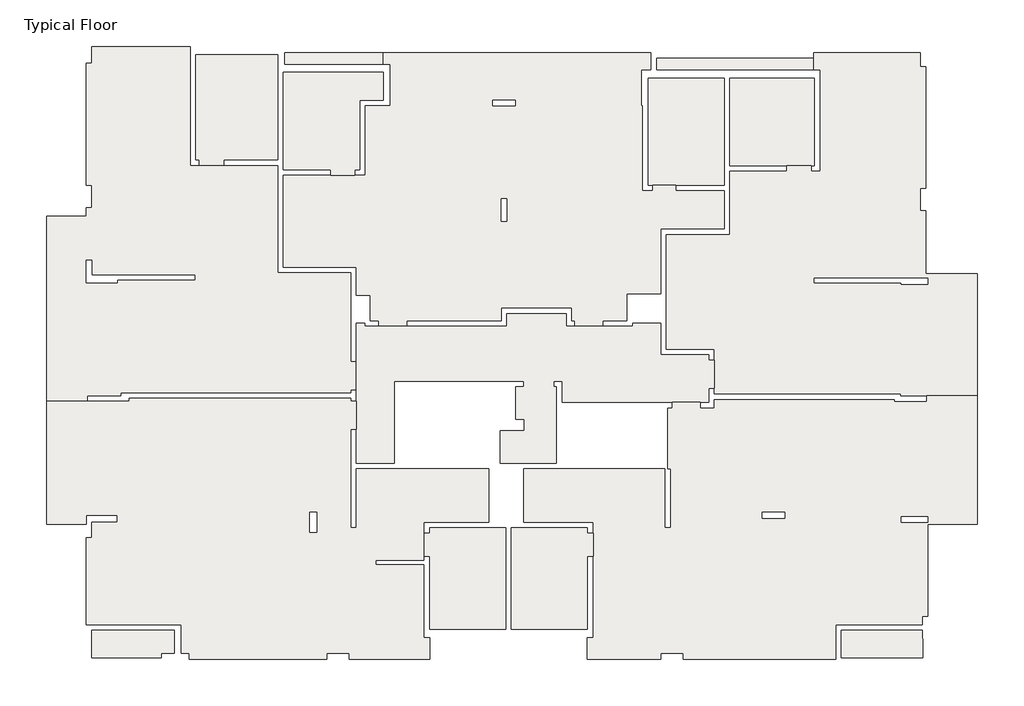
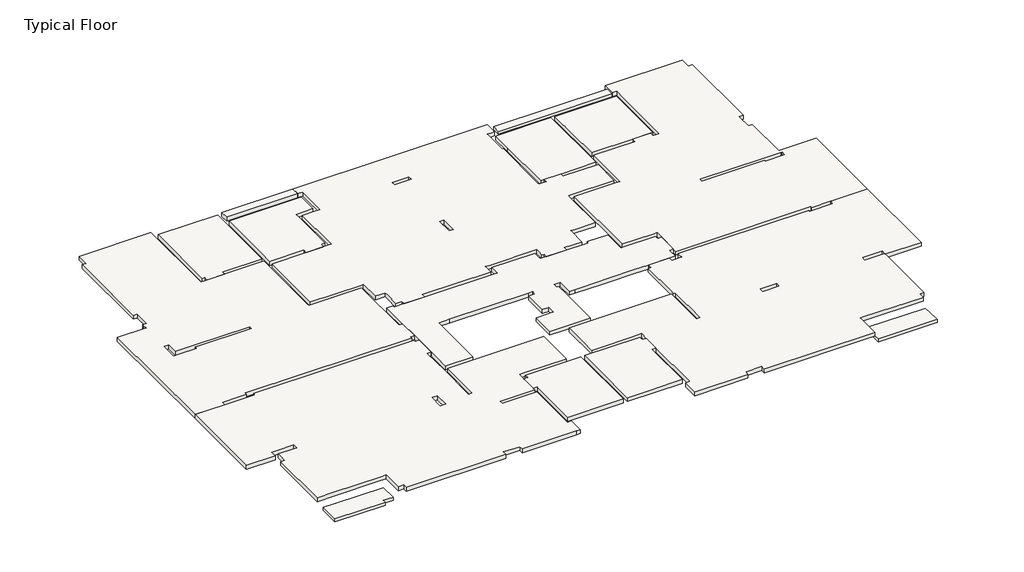
# One storey: 16 slabs.
"""IFC4 building model written with IfcOpenShell, lengths in millimetres."""

import ifcopenshell
import ifcopenshell.guid

model = None  # the IFC model being written
_history = None  # IfcOwnerHistory: only IFC2X3 demands one
_inside = {}  # id of a spatial element -> (the spatial element, [elements in it])
_under = {}  # id of a project, library or spatial element -> (it, [spatial elements below it])
_declared = {}  # id of a project -> (the project, [libraries it declares])
_typed = {}  # id of a type object -> (the type object, [elements of that type])
_made_of = {}  # id of a material, layer set ... -> (it, [elements and type objects made of it])


def new_model(schema):
    """Start an empty IFC model of exactly this schema.

    Asked for "IFC4X3", IfcOpenShell would pick the latest addendum, in which some entities
    have other attributes; the version numbers below select the first issue.
    IFC2X3 requires an IfcOwnerHistory on every rooted entity: one is made here for all.
    """
    global model, _history
    if schema == "IFC4X3":
        model = ifcopenshell.file(schema_version=(4, 3, 0, 0))
    else:
        model = ifcopenshell.file(schema=schema)
    _inside.clear()
    _under.clear()
    _declared.clear()
    _typed.clear()
    _made_of.clear()
    _history = None
    if model.schema == "IFC2X3":
        org = make("IfcOrganization", Name="unknown")
        user = make(
            "IfcPersonAndOrganization",
            ThePerson=make("IfcPerson", FamilyName="unknown"),
            TheOrganization=org,
        )
        app = make(
            "IfcApplication",
            ApplicationDeveloper=org,
            Version="unknown",
            ApplicationFullName="unknown",
            ApplicationIdentifier="unknown",
        )
        _history = make(
            "IfcOwnerHistory",
            OwningUser=user,
            OwningApplication=app,
            ChangeAction="ADDED",
            CreationDate=0,
        )
    return model


def make(cls, **values):
    """One entity of the class cls with the attributes given. An attribute that is None is left unset."""
    return model.create_entity(
        cls, **{name: value for name, value in values.items() if value is not None}
    )


def rooted(cls, **values):
    """An entity with a GlobalId (a new one), such as an element, a storey or a relation."""
    return make(cls, GlobalId=ifcopenshell.guid.new(), OwnerHistory=_history, **values)


def si_unit(unit_type, name, prefix=None):
    """IfcSIUnit, for example si_unit("LENGTHUNIT", "METRE", prefix="MILLI")."""
    return make("IfcSIUnit", UnitType=unit_type, Prefix=prefix, Name=name)


def assignment(units):
    """IfcUnitAssignment: the units of a project."""
    return None if units is None else make("IfcUnitAssignment", Units=units)


def point(xyz):
    """IfcCartesianPoint."""
    return None if xyz is None else make("IfcCartesianPoint", Coordinates=xyz)


def direction(xyz):
    """IfcDirection."""
    return None if xyz is None else make("IfcDirection", DirectionRatios=xyz)


def frame(location, z_axis=None, x_axis=None):
    """IfcAxis2Placement3D, a coordinate frame: its origin and axes. An axis left out is left unset."""
    return make(
        "IfcAxis2Placement3D",
        Location=point(location),
        Axis=direction(z_axis),
        RefDirection=direction(x_axis),
    )


def origin():
    """The frame at (0, 0, 0) with its axes left unset."""
    return frame((0.0, 0.0, 0.0))


def place(relative_to, where):
    """IfcLocalPlacement: puts the frame where relative to a parent placement (None: the world)."""
    return make(
        "IfcLocalPlacement", PlacementRelTo=relative_to, RelativePlacement=where
    )


def context(
    kind, dimensions, precision=None, world=None, true_north=None, identifier=None
):
    """IfcGeometricRepresentationContext, for example the 3D "Model" context."""
    return make(
        "IfcGeometricRepresentationContext",
        ContextIdentifier=identifier,
        ContextType=kind,
        CoordinateSpaceDimension=dimensions,
        Precision=precision,
        WorldCoordinateSystem=world,
        TrueNorth=true_north,
    )


def project(units=None, contexts=None):
    """IfcProject with its units and contexts."""
    return rooted(
        "IfcProject",
        Name="project",
        RepresentationContexts=contexts,
        UnitsInContext=assignment(units),
    )


def spatial(cls, under=None, at=None, **own):
    """A site, building, storey or space (cls), placed at a placement, below another one or the project."""
    s = rooted(cls, ObjectPlacement=at, **own)
    if under is not None:
        _under.setdefault(under.id(), (under, []))[1].append(s)
    return s


def polyline(points):
    """IfcPolyline through the points."""
    return make("IfcPolyline", Points=[point(p) for p in points])


def outline(outer, holes=None, kind="AREA"):
    """IfcArbitraryClosedProfileDef: a profile drawn as a closed curve; with holes, ...WithVoids."""
    if holes is None:
        return make("IfcArbitraryClosedProfileDef", ProfileType=kind, OuterCurve=outer)
    return make(
        "IfcArbitraryProfileDefWithVoids",
        ProfileType=kind,
        OuterCurve=outer,
        InnerCurves=holes,
    )


def extrude(swept, where, along, depth):
    """IfcExtrudedAreaSolid: the profile swept, set in the frame where, extruded along a direction by depth."""
    return make(
        "IfcExtrudedAreaSolid",
        SweptArea=swept,
        Position=where,
        ExtrudedDirection=direction(along),
        Depth=depth,
    )


def faces_of(points, faces, orient=None, outer=None):
    """IfcFace entities. A face is a list of loops; a loop is a list of indices into points, from 0.

    orient and outer hold one flag for each loop. By default every Orientation is true, the
    first loop of a face is its IfcFaceOuterBound and the others are IfcFaceBound.
    """
    made = []
    for i, loops in enumerate(faces):
        bounds = []
        for j, loop in enumerate(loops):
            is_outer = j == 0 if outer is None else outer[i][j]
            bounds.append(
                make(
                    "IfcFaceOuterBound" if is_outer else "IfcFaceBound",
                    Bound=make("IfcPolyLoop", Polygon=[points[k] for k in loop]),
                    Orientation=True if orient is None else orient[i][j],
                )
            )
        made.append(make("IfcFace", Bounds=bounds))
    return made


def faceted_brep(points, faces, orient=None, outer=None, voids=None):
    """IfcFacetedBrep: a solid bounded by flat faces; with voids (closed shells), ...WithVoids."""
    shared = [point(p) for p in points]
    hull = make("IfcClosedShell", CfsFaces=faces_of(shared, faces, orient, outer))
    if voids is None:
        return make("IfcFacetedBrep", Outer=hull)
    return make(
        "IfcFacetedBrepWithVoids",
        Outer=hull,
        Voids=[
            make(cls, CfsFaces=faces_of(shared, fs, o, b)) for cls, fs, o, b in voids
        ],
    )


def shape(context_of_items, identifier, shape_type, items):
    """IfcShapeRepresentation: the items that make up one representation, for example the "Body"."""
    return make(
        "IfcShapeRepresentation",
        ContextOfItems=context_of_items,
        RepresentationIdentifier=identifier,
        RepresentationType=shape_type,
        Items=items,
    )


def made_of(thing, what):
    """Note that an element or type object is made of a material, layer set ...; save() writes the relation."""
    if what is not None:
        _made_of.setdefault(what.id(), (what, []))[1].append(thing)
    return thing


def element(
    cls,
    number,
    at=None,
    inside=None,
    cuts=None,
    type_object=None,
    material=None,
    context=None,
    identifier="Body",
    shape_type=None,
    held_by="IfcProductDefinitionShape",
    body=None,
    shapes=None,
    **own,
):
    """One element of the class cls, such as IfcWall. Its Tag is "e" and its number.

    at: its placement. inside: the storey or other place that contains it. cuts: it is an
    opening in that element (IfcRelVoidsElement). A single representation is given by context,
    identifier, shape_type and body (its items); several are given by shapes. held_by: the class
    of the entity that holds the representations. save() writes the other relations.
    """
    e = rooted(cls, Tag="e%d" % number, ObjectPlacement=at, **own)
    if body is not None:
        shapes = [shape(context, identifier, shape_type, body)]
    if shapes is not None:
        e.Representation = make(held_by, Representations=shapes)
    if inside is not None:
        _inside.setdefault(inside.id(), (inside, []))[1].append(e)
    if cuts is not None:
        rooted(
            "IfcRelVoidsElement", RelatingBuildingElement=cuts, RelatedOpeningElement=e
        )
    if type_object is not None:
        _typed.setdefault(type_object.id(), (type_object, []))[1].append(e)
    return made_of(e, material)


def aggregate(whole, parts):
    """IfcRelAggregates: a whole, such as a stair, and the parts it consists of."""
    return rooted("IfcRelAggregates", RelatingObject=whole, RelatedObjects=parts)


def save(model, path):
    """Write the relations noted so far, then the file.

    IfcRelAggregates (storeys below a building ...), IfcRelContainedInSpatialStructure (elements
    in a storey), IfcRelDefinesByType, IfcRelAssociatesMaterial and IfcRelDeclares: one each for
    every whole, place, type object, material and project.
    """
    for whole, parts in _under.values():
        aggregate(whole, parts)
    for where, things in _inside.values():
        rooted(
            "IfcRelContainedInSpatialStructure",
            RelatedElements=things,
            RelatingStructure=where,
        )
    for kind, things in _typed.values():
        rooted("IfcRelDefinesByType", RelatedObjects=things, RelatingType=kind)
    for what, things in _made_of.values():
        rooted("IfcRelAssociatesMaterial", RelatedObjects=things, RelatingMaterial=what)
    for by, libraries in _declared.values():
        rooted("IfcRelDeclares", RelatingContext=by, RelatedDefinitions=libraries)
    model.write(path)


model = new_model("IFC4")

# Units and contexts
model_context = context("Model", 3, world=origin())
ifc_project = project(units=[si_unit("LENGTHUNIT", "METRE", prefix="MILLI")], contexts=[model_context])

# Site, building, storey
site = spatial("IfcSite", under=ifc_project)
building = spatial("IfcBuilding", under=site)
storey = spatial("IfcBuildingStorey", under=building, Name="Typical Floor", Elevation=3270.0)

# Slabs
placement = place(None, origin())
element("IfcSlab", 1, ObjectType="15", at=placement, inside=storey, context=model_context, shape_type="Brep", body=[
    faceted_brep([(-21571.9643546, 17066.3078446, 2670.0), (-24032.496199, 17066.3078446, 2670.0), (-24034.296226, 17066.3078446, 2670.0), (-24034.296226, 18036.7796078, 2670.0), (-23432.496199, 18036.7796078, 2670.0), (-23432.496199, 18038.5478478, 2670.0), (-21102.3452666, 18038.5478478, 2670.0), (-21102.3452666, 17215.5200253, 2670.0), (-21571.9643546, 17215.5200253, 2670.0), (-24034.296226, 17066.3078446, 2820.0), (-24032.496199, 17066.3078446, 2820.0), (-21571.9643546, 17066.3078446, 2820.0), (-21571.9643546, 17215.5200253, 2820.0), (-21102.3452666, 17215.5200253, 2820.0), (-21102.3452666, 18036.7796078, 2820.0), (-21102.3452666, 18038.5478478, 2820.0), (-23432.496199, 18038.5478478, 2820.0), (-23432.496199, 18036.7796078, 2820.0), (-24032.496199, 18036.7796078, 2820.0), (-24034.296226, 18036.7796078, 2820.0)], [[[0, 1, 2, 3, 4, 5, 6, 7, 8]], [[9, 10, 11, 12, 13, 14, 15, 16, 17, 18, 19]], [[11, 0, 8, 12]], [[2, 1, 0, 11, 10, 9]], [[2, 9, 19, 3]], [[15, 6, 5, 16]], [[7, 6, 15, 14, 13]], [[12, 8, 7, 13]], [[4, 17, 16, 5]], [[17, 4, 3, 19, 18]]]),
])
element("IfcSlab", 2, ObjectType="15", at=placement, inside=storey, context=model_context, shape_type="Brep", body=[
    faceted_brep([(5430.732608, 17066.3078446, 2670.0), (5420.732608, 17066.3078446, 2670.0), (2546.318889, 17066.3078446, 2670.0), (2541.318889, 17066.3078446, 2670.0), (2541.318889, 17435.7075634, 2670.0), (2546.318889, 17435.7075634, 2670.0), (2546.318889, 18040.7075634, 2670.0), (5420.732608, 18040.7075634, 2670.0), (5420.732608, 17735.2006534, 2670.0), (5430.732608, 17735.2006534, 2670.0), (2541.318889, 17066.3078446, 2820.0), (2546.318889, 17066.3078446, 2820.0), (5420.732608, 17066.3078446, 2820.0), (5430.732608, 17066.3078446, 2820.0), (5430.732608, 17735.2006534, 2820.0), (5420.732608, 17735.2006534, 2820.0), (5420.732608, 18035.7075634, 2820.0), (5420.732608, 18040.7075634, 2820.0), (2546.318889, 18040.7075634, 2820.0), (2546.318889, 18035.7075634, 2820.0), (2546.318889, 17435.7075634, 2820.0), (2541.318889, 17435.7075634, 2820.0)], [[[0, 1, 2, 3, 4, 5, 6, 7, 8, 9]], [[10, 11, 12, 13, 14, 15, 16, 17, 18, 19, 20, 21]], [[3, 2, 1, 0, 13, 12, 11, 10]], [[3, 10, 21, 4]], [[6, 18, 17, 7]], [[13, 0, 9, 14]], [[5, 20, 19, 18, 6]], [[20, 5, 4, 21]], [[8, 15, 14, 9]], [[15, 8, 7, 17, 16]]]),
])
element("IfcSlab", 3, ObjectType="15", at=placement, inside=storey, context=model_context, shape_type="SweptSolid", body=[
    extrude(outline(polyline([(1566.3525769, 38314.4998391), (1566.3525769, 37914.469069), (-4002.3443382, 37914.469069), (-4002.3443382, 38314.4998391), (1566.3525769, 38314.4998391)])), frame((0.0, 0.0, 3070.0), z_axis=(0.0, 0.0, 1.0), x_axis=(1.0, 0.0, 0.0)), (0.0, 0.0, 1.0), 150.0),
])
element("IfcSlab", 4, ObjectType="20", at=placement, inside=storey, context=model_context, shape_type="Brep", body=[
    faceted_brep([(1597.1133398, 37614.469069, 3070.0), (1597.1133398, 34516.3054573, 3070.0), (1475.3435315, 34516.3054573, 3070.0), (620.1311917, 34516.3054573, 3070.0), (-1403.2009922, 34516.3054573, 3070.0), (-1403.2009922, 37614.469069, 3070.0), (1597.1133398, 37614.469069, 3270.0), (-1403.2009922, 37614.469069, 3270.0), (-1403.2009922, 34516.3054573, 3270.0), (620.1311917, 34516.3054573, 3270.0), (1475.3435315, 34516.3054573, 3270.0), (1597.1133398, 34516.3054573, 3270.0)], [[[0, 1, 2, 3, 4, 5]], [[6, 7, 8, 9, 10, 11]], [[1, 0, 6, 11]], [[4, 3, 2, 1, 11, 10, 9, 8]], [[5, 4, 8, 7]], [[0, 5, 7, 6]]]),
])
element("IfcSlab", 5, ObjectType="20", at=placement, inside=storey, context=model_context, shape_type="Brep", body=[
    faceted_brep([(-1603.2009922, 37614.469069, 3070.0), (-1603.2009922, 33815.7403229, 3070.0), (-3320.8331575, 33815.7403229, 3070.0), (-4138.8749491, 33815.7403229, 3070.0), (-4301.8715139, 33815.7403229, 3070.0), (-4301.8715139, 36636.0817113, 3070.0), (-4302.6593333, 36636.0817113, 3070.0), (-4302.6593333, 37614.469069, 3070.0), (-1603.2009922, 33815.7403229, 3270.0), (-1603.2009922, 37614.469069, 3270.0), (-4302.6593333, 37614.469069, 3270.0), (-4302.6593333, 36636.0817113, 3270.0), (-4301.8715139, 36636.0817113, 3270.0), (-4301.8715139, 33815.7403229, 3270.0), (-4138.8749491, 33815.7403229, 3270.0), (-3320.8331575, 33815.7403229, 3270.0)], [[[0, 1, 2, 3, 4, 5, 6, 7]], [[8, 9, 10, 11, 12, 13, 14, 15]], [[1, 0, 9, 8]], [[1, 8, 15, 14, 13, 4, 3, 2]], [[10, 7, 6, 11]], [[0, 7, 10, 9]], [[12, 5, 4, 13]], [[5, 12, 11, 6]]]),
])
element("IfcSlab", 6, ObjectType="20", at=placement, inside=storey, context=model_context, shape_type="Brep", body=[
    faceted_brep([(1566.3525769, 37914.469069, 3070.0), (1566.3525769, 38314.4998391, 3070.0), (1566.3525769, 38515.575292, 3070.0), (5346.4978686, 38515.575292, 3070.0), (5346.4978686, 38016.0787934, 3070.0), (5546.4978686, 38016.0787934, 3070.0), (5546.4978686, 33715.2026429, 3070.0), (5346.4978686, 33715.2026429, 3070.0), (5346.4978686, 32915.2026429, 3070.0), (5546.4978686, 32915.2026429, 3070.0), (5546.4978686, 30686.4079799, 3070.0), (5547.5722379, 30686.4079799, 3070.0), (7376.2745907, 30686.4079799, 3070.0), (7376.2745907, 26346.3859634, 3070.0), (5607.1364173, 26346.3859634, 3070.0), (5577.2268706, 26346.3859634, 3070.0), (4656.569824, 26346.3859634, 3070.0), (4656.569824, 26415.1864621, 3070.0), (-1953.6864162, 26415.1864621, 3070.0), (-1953.6864162, 26616.2585064, 3070.0), (-1953.6864162, 27615.2787722, 3070.0), (-1953.6864162, 28004.6755732, 3070.0), (-2153.6864162, 28004.6755732, 3070.0), (-3652.0941989, 28004.6755732, 3070.0), (-3652.0941989, 32066.405062, 3070.0), (-1603.2009922, 32066.405062, 3070.0), (-1403.2009922, 32066.405062, 3070.0), (-1403.2009922, 34316.3054573, 3070.0), (620.1311917, 34316.3054573, 3070.0), (620.1311917, 34516.3054573, 3070.0), (1475.3435315, 34516.3054573, 3070.0), (1475.3435315, 34316.3054573, 3070.0), (1797.1133398, 34316.3054573, 3070.0), (1797.1133398, 34516.3054573, 3070.0), (1797.1133398, 37614.469069, 3070.0), (1797.1133398, 37914.469069, 3070.0), (1598.0523567, 30514.7063432, 3070.0), (1598.0523567, 30364.7063432, 3070.0), (4667.1364173, 30364.7063432, 3070.0), (4667.1364173, 30314.7063432, 3070.0), (5607.1364173, 30314.7063432, 3070.0), (5607.1364173, 30514.7063432, 3070.0), (5546.4978686, 30514.7063432, 3070.0), (4667.1364173, 30514.7063432, 3070.0), (1566.3525769, 38515.575292, 3270.0), (1566.3525769, 37914.469069, 3270.0), (1797.1133398, 37914.469069, 3270.0), (1797.1133398, 37614.469069, 3270.0), (1797.1133398, 34516.3054573, 3270.0), (1797.1133398, 34316.3054573, 3270.0), (1475.3435315, 34316.3054573, 3270.0), (1475.3435315, 34516.3054573, 3270.0), (620.1311917, 34516.3054573, 3270.0), (620.1311917, 34316.3054573, 3270.0), (-1403.2009922, 34316.3054573, 3270.0), (-1403.2009922, 32066.405062, 3270.0), (-1603.2009922, 32066.405062, 3270.0), (-3652.0941989, 32066.405062, 3270.0), (-3652.0941989, 28004.6755732, 3270.0), (-2153.6864162, 28004.6755732, 3270.0), (-1953.6864162, 28004.6755732, 3270.0), (-1953.6864162, 27615.2787722, 3270.0), (-1953.6864162, 26616.2585064, 3270.0), (-1953.6864162, 26415.1864621, 3270.0), (4656.569824, 26415.1864621, 3270.0), (4656.569824, 26346.3859634, 3270.0), (5577.2268706, 26346.3859634, 3270.0), (5607.1364173, 26346.3859634, 3270.0), (7376.2745907, 26346.3859634, 3270.0), (7376.2745907, 30686.4079799, 3270.0), (5546.4978686, 30686.4079799, 3270.0), (5546.4978686, 32915.2026429, 3270.0), (5346.4978686, 32915.2026429, 3270.0), (5346.4978686, 33715.2026429, 3270.0), (5546.4978686, 33715.2026429, 3270.0), (5546.4978686, 38016.0787934, 3270.0), (5346.4978686, 38016.0787934, 3270.0), (5346.4978686, 38515.575292, 3270.0), (1598.0523567, 30364.7063432, 3270.0), (1598.0523567, 30514.7063432, 3270.0), (4667.1364173, 30514.7063432, 3270.0), (5546.4978686, 30514.7063432, 3270.0), (5607.1364173, 30514.7063432, 3270.0), (5607.1364173, 30314.7063432, 3270.0), (4667.1364173, 30314.7063432, 3270.0), (4667.1364173, 30364.7063432, 3270.0), (1566.3525769, 37914.469069, 3220.0)], [[[0, 1, 2, 3, 4, 5, 6, 7, 8, 9, 10, 11, 12, 13, 14, 15, 16, 17, 18, 19, 20, 21, 22, 23, 24, 25, 26, 27, 28, 29, 30, 31, 32, 33, 34, 35], [36, 37, 38, 39, 40, 41, 42, 43]], [[44, 45, 46, 47, 48, 49, 50, 51, 52, 53, 54, 55, 56, 57, 58, 59, 60, 61, 62, 63, 64, 65, 66, 67, 68, 69, 70, 71, 72, 73, 74, 75, 76, 77], [78, 79, 80, 81, 82, 83, 84, 85]], [[2, 1, 0, 86, 45, 44]], [[3, 2, 44, 77]], [[4, 3, 77, 76]], [[5, 4, 76, 75]], [[6, 5, 75, 74]], [[7, 6, 74, 73]], [[8, 7, 73, 72]], [[9, 8, 72, 71]], [[10, 9, 71, 70]], [[79, 36, 43, 42, 81, 80]], [[37, 36, 79, 78]], [[38, 37, 78, 85]], [[39, 38, 85, 84]], [[40, 39, 84, 83]], [[16, 15, 14, 67, 66, 65]], [[17, 16, 65, 64]], [[18, 17, 64, 63]], [[19, 18, 63, 62]], [[20, 19, 62, 61]], [[21, 20, 61, 60]], [[21, 60, 59, 58, 23, 22]], [[24, 23, 58, 57]], [[24, 57, 56, 55, 26, 25]], [[27, 26, 55, 54]], [[28, 27, 54, 53]], [[29, 28, 53, 52]], [[30, 29, 52, 51]], [[31, 30, 51, 50]], [[32, 31, 50, 49]], [[32, 49, 48, 47, 46, 35, 34, 33]], [[0, 35, 46, 45, 86]], [[12, 11, 10, 70, 69]], [[13, 12, 69, 68]], [[14, 13, 68, 67]], [[41, 40, 83, 82]], [[42, 41, 82, 81]]]),
])
element("IfcSlab", 7, ObjectType="20", at=placement, inside=storey, context=model_context, shape_type="Brep", body=[
    faceted_brep([(-1953.6864162, 27615.2787722, 3070.0), (-1953.6864162, 26616.2585064, 3070.0), (-2153.6864162, 26616.2585064, 3070.0), (-2153.6864162, 26116.7313306, 3070.0), (-2453.0431631, 26116.7313306, 3070.0), (-3452.0634289, 26116.7313306, 3070.0), (-4152.6285632, 26116.7313306, 3070.0), (-5452.2172791, 26116.7313306, 3070.0), (-5750.6383247, 26116.7313306, 3070.0), (-7052.3403593, 26116.7313306, 3070.0), (-7352.8747236, 26116.7313306, 3070.0), (-7352.8747236, 26666.0050514, 3070.0), (-7352.8747236, 26866.0050514, 3070.0), (-7653.4431737, 26866.0050514, 3070.0), (-7653.4431737, 26666.0050514, 3070.0), (-7552.8747236, 26666.0050514, 3070.0), (-7552.8747236, 26116.7313306, 3070.0), (-7552.8747236, 25916.7313306, 3070.0), (-7552.8747236, 23965.2552968, 3070.0), (-9538.2512588, 23965.2552968, 3070.0), (-9538.2512588, 25114.9330071, 3070.0), (-8698.2512588, 25114.9330071, 3070.0), (-8698.2512588, 25514.9330071, 3070.0), (-9003.2512588, 25514.9330071, 3070.0), (-9003.2512588, 26664.9330071, 3070.0), (-8703.2512588, 26664.9330071, 3070.0), (-8703.2512588, 26864.9330071, 3070.0), (-8902.548455, 26864.9330071, 3070.0), (-12762.548455, 26864.9330071, 3070.0), (-13303.2512588, 26864.9330071, 3070.0), (-13303.2512588, 26664.9330071, 3070.0), (-13302.548455, 26664.9330071, 3070.0), (-13302.548455, 23965.2552968, 3070.0), (-14651.8837159, 23965.2552968, 3070.0), (-14651.8837159, 25164.3063326, 3070.0), (-14652.9249902, 25164.3063326, 3070.0), (-14652.9249902, 26165.4399171, 3070.0), (-14652.9249902, 26561.209964, 3070.0), (-14652.9249902, 27566.6042716, 3070.0), (-14652.9249902, 28915.3710824, 3070.0), (-14353.3978144, 28915.3710824, 3070.0), (-14353.3978144, 28815.3710824, 3070.0), (-13852.8634501, 28815.3710824, 3070.0), (-12851.7298656, 28815.3710824, 3070.0), (-9317.0680709, 28815.3710824, 3070.0), (-9317.0680709, 29015.3710824, 3070.0), (-9317.0680709, 29265.1483974, 3070.0), (-7203.6658586, 29265.1483974, 3070.0), (-7203.6658586, 29015.3710824, 3070.0), (-7203.6658586, 28815.3710824, 3070.0), (-6902.0561342, 28815.3710824, 3070.0), (-5903.0358684, 28815.3710824, 3070.0), (-4853.2277833, 28815.3710824, 3070.0), (-4853.2277833, 28914.6755732, 3070.0), (-3852.0941989, 28914.6755732, 3070.0), (-3852.0941989, 27804.6755732, 3070.0), (-3652.0941989, 27804.6755732, 3070.0), (-2153.6864162, 27804.6755732, 3070.0), (-2153.6864162, 27615.2787722, 3070.0), (-1953.6864162, 26616.2585064, 3270.0), (-1953.6864162, 27615.2787722, 3270.0), (-2153.6864162, 27615.2787722, 3270.0), (-2153.6864162, 27804.6755732, 3270.0), (-3652.0941989, 27804.6755732, 3270.0), (-3852.0941989, 27804.6755732, 3270.0), (-3852.0941989, 28914.6755732, 3270.0), (-4853.2277833, 28914.6755732, 3270.0), (-4853.2277833, 28815.3710824, 3270.0), (-5903.0358684, 28815.3710824, 3270.0), (-6902.0561342, 28815.3710824, 3270.0), (-7203.6658586, 28815.3710824, 3270.0), (-7203.6658586, 29015.3710824, 3270.0), (-7203.6658586, 29265.1483974, 3270.0), (-9317.0680709, 29265.1483974, 3270.0), (-9317.0680709, 29015.3710824, 3270.0), (-9317.0680709, 28815.3710824, 3270.0), (-12851.7298656, 28815.3710824, 3270.0), (-13852.8634501, 28815.3710824, 3270.0), (-14353.3978144, 28815.3710824, 3270.0), (-14353.3978144, 28915.3710824, 3270.0), (-14652.9249902, 28915.3710824, 3270.0), (-14652.9249902, 27566.6042716, 3270.0), (-14652.9249902, 26561.209964, 3270.0), (-14652.9249902, 26165.4399171, 3270.0), (-14652.9249902, 25164.3063326, 3270.0), (-14651.8837159, 25164.3063326, 3270.0), (-14651.8837159, 23965.2552968, 3270.0), (-13302.548455, 23965.2552968, 3270.0), (-13302.548455, 26664.9330071, 3270.0), (-13303.2512588, 26664.9330071, 3270.0), (-13303.2512588, 26864.9330071, 3270.0), (-12762.548455, 26864.9330071, 3270.0), (-8902.548455, 26864.9330071, 3270.0), (-8703.2512588, 26864.9330071, 3270.0), (-8703.2512588, 26664.9330071, 3270.0), (-9003.2512588, 26664.9330071, 3270.0), (-9003.2512588, 25514.9330071, 3270.0), (-8698.2512588, 25514.9330071, 3270.0), (-8698.2512588, 25114.9330071, 3270.0), (-9538.2512588, 25114.9330071, 3270.0), (-9538.2512588, 23965.2552968, 3270.0), (-7552.8747236, 23965.2552968, 3270.0), (-7552.8747236, 25916.7313306, 3270.0), (-7552.8747236, 26116.7313306, 3270.0), (-7552.8747236, 26666.0050514, 3270.0), (-7653.4431737, 26666.0050514, 3270.0), (-7653.4431737, 26866.0050514, 3270.0), (-7352.8747236, 26866.0050514, 3270.0), (-7352.8747236, 26666.0050514, 3270.0), (-7352.8747236, 26116.7313306, 3270.0), (-7052.3403593, 26116.7313306, 3270.0), (-5750.6383247, 26116.7313306, 3270.0), (-5452.2172791, 26116.7313306, 3270.0), (-4152.6285632, 26116.7313306, 3270.0), (-3452.0634289, 26116.7313306, 3270.0), (-2453.0431631, 26116.7313306, 3270.0), (-2153.6864162, 26116.7313306, 3270.0), (-2153.6864162, 26616.2585064, 3270.0)], [[[0, 1, 2, 3, 4, 5, 6, 7, 8, 9, 10, 11, 12, 13, 14, 15, 16, 17, 18, 19, 20, 21, 22, 23, 24, 25, 26, 27, 28, 29, 30, 31, 32, 33, 34, 35, 36, 37, 38, 39, 40, 41, 42, 43, 44, 45, 46, 47, 48, 49, 50, 51, 52, 53, 54, 55, 56, 57, 58]], [[59, 60, 61, 62, 63, 64, 65, 66, 67, 68, 69, 70, 71, 72, 73, 74, 75, 76, 77, 78, 79, 80, 81, 82, 83, 84, 85, 86, 87, 88, 89, 90, 91, 92, 93, 94, 95, 96, 97, 98, 99, 100, 101, 102, 103, 104, 105, 106, 107, 108, 109, 110, 111, 112, 113, 114, 115, 116, 117]], [[1, 0, 60, 59]], [[2, 1, 59, 117]], [[3, 2, 117, 116]], [[3, 116, 115, 114, 5, 4]], [[5, 114, 113, 112, 111, 110, 9, 8, 7, 6]], [[10, 9, 110, 109]], [[10, 109, 108, 107, 12, 11]], [[13, 12, 107, 106]], [[14, 13, 106, 105]], [[15, 14, 105, 104]], [[15, 104, 103, 102, 101, 18, 17, 16]], [[19, 18, 101, 100]], [[20, 19, 100, 99]], [[21, 20, 99, 98]], [[22, 21, 98, 97]], [[23, 22, 97, 96]], [[24, 23, 96, 95]], [[25, 24, 95, 94]], [[26, 25, 94, 93]], [[27, 26, 93, 92]], [[28, 27, 92, 91]], [[28, 91, 90, 29]], [[87, 32, 31, 88]], [[33, 32, 87, 86]], [[34, 33, 86, 85]], [[35, 34, 85, 84]], [[36, 35, 84, 83]], [[37, 36, 83, 82]], [[38, 37, 82, 81]], [[39, 38, 81, 80]], [[40, 39, 80, 79]], [[41, 40, 79, 78]], [[42, 41, 78, 77]], [[43, 42, 77, 76]], [[44, 43, 76, 75]], [[44, 75, 74, 73, 46, 45]], [[47, 46, 73, 72]], [[47, 72, 71, 70, 49, 48]], [[50, 49, 70, 69]], [[51, 50, 69, 68]], [[52, 51, 68, 67]], [[53, 52, 67, 66]], [[54, 53, 66, 65]], [[55, 54, 65, 64]], [[55, 64, 63, 62, 57, 56]], [[58, 57, 62, 61]], [[0, 58, 61, 60]], [[30, 89, 88, 31]], [[29, 90, 89, 30]]]),
])
element("IfcSlab", 8, ObjectType="20", at=placement, inside=storey, context=model_context, shape_type="Brep", body=[
    faceted_brep([(-13700.7193614, 37815.0067491, 3070.0), (-13700.7193614, 36836.0817113, 3070.0), (-14532.2613121, 36836.0817113, 3070.0), (-14532.2613121, 36636.0817113, 3070.0), (-14532.2613121, 34366.055318, 3070.0), (-14705.8261281, 34366.055318, 3070.0), (-14705.8261281, 34166.055318, 3070.0), (-15560.9362106, 34166.055318, 3070.0), (-15560.9362106, 34366.055318, 3070.0), (-17231.9731082, 34366.055318, 3070.0), (-17231.9731082, 37815.0067491, 3070.0), (-13700.7193614, 36836.0817113, 3270.0), (-13700.7193614, 37815.0067491, 3270.0), (-17231.9731082, 37815.0067491, 3270.0), (-17231.9731082, 34366.055318, 3270.0), (-15560.9362106, 34366.055318, 3270.0), (-15560.9362106, 34166.055318, 3270.0), (-14705.8261281, 34166.055318, 3270.0), (-14705.8261281, 34366.055318, 3270.0), (-14532.2613121, 34366.055318, 3270.0), (-14532.2613121, 36636.0817113, 3270.0), (-14532.2613121, 36836.0817113, 3270.0)], [[[0, 1, 2, 3, 4, 5, 6, 7, 8, 9, 10]], [[11, 12, 13, 14, 15, 16, 17, 18, 19, 20, 21]], [[1, 0, 12, 11]], [[2, 1, 11, 21]], [[2, 21, 20, 19, 4, 3]], [[5, 4, 19, 18]], [[6, 5, 18, 17]], [[7, 6, 17, 16]], [[8, 7, 16, 15]], [[9, 8, 15, 14]], [[10, 9, 14, 13]], [[0, 10, 13, 12]]]),
])
element("IfcSlab", 9, ObjectType="20", at=placement, inside=storey, context=model_context, shape_type="Brep", body=[
    faceted_brep([(-13700.7193614, 38514.5374263, 3070.0), (-4202.3443382, 38514.5374263, 3070.0), (-4202.3443382, 37914.469069, 3070.0), (-4302.6593333, 37914.469069, 3070.0), (-4552.6593333, 37914.469069, 3070.0), (-4552.6593333, 36636.0817113, 3070.0), (-4501.8715139, 36636.0817113, 3070.0), (-4501.8715139, 33815.7403229, 3070.0), (-4501.8715139, 33615.7403229, 3070.0), (-4138.8749491, 33615.7403229, 3070.0), (-4138.8749491, 33815.7403229, 3070.0), (-3320.8331575, 33815.7403229, 3070.0), (-3320.8331575, 33615.7403229, 3070.0), (-1603.2009922, 33615.7403229, 3070.0), (-1603.2009922, 32266.405062, 3070.0), (-3852.0941989, 32266.405062, 3070.0), (-3852.0941989, 32066.405062, 3070.0), (-3852.0941989, 29964.6755732, 3070.0), (-4853.2277833, 29964.6755732, 3070.0), (-5053.2277833, 29964.6755732, 3070.0), (-5053.2277833, 29015.3710824, 3070.0), (-5903.0358684, 29015.3710824, 3070.0), (-5903.0358684, 28815.3710824, 3070.0), (-6902.0561342, 28815.3710824, 3070.0), (-6902.0561342, 29015.3710824, 3070.0), (-7003.6658586, 29015.3710824, 3070.0), (-7003.6658586, 29265.1483974, 3070.0), (-7003.6658586, 29465.1483974, 3070.0), (-9317.0680709, 29465.1483974, 3070.0), (-9517.0680709, 29465.1483974, 3070.0), (-9517.0680709, 29015.3710824, 3070.0), (-12851.7298656, 29015.3710824, 3070.0), (-12851.7298656, 28815.3710824, 3070.0), (-13852.8634501, 28815.3710824, 3070.0), (-13852.8634501, 29015.3710824, 3070.0), (-14153.3978144, 29015.3710824, 3070.0), (-14153.3978144, 29714.8949424, 3070.0), (-14153.3978144, 29914.8949424, 3070.0), (-14652.9249902, 29914.8949424, 3070.0), (-14652.9249902, 30914.9872525, 3070.0), (-14852.9249902, 30914.9872525, 3070.0), (-17231.9731082, 30914.9872525, 3070.0), (-17231.9731082, 34166.055318, 3070.0), (-15560.9362106, 34166.055318, 3070.0), (-14705.8261281, 34166.055318, 3070.0), (-14332.2613121, 34166.055318, 3070.0), (-14332.2613121, 34366.055318, 3070.0), (-14332.2613121, 36636.0817113, 3070.0), (-13700.7193614, 36636.0817113, 3070.0), (-13450.7193614, 36636.0817113, 3070.0), (-13450.7193614, 37815.0067491, 3070.0), (-13450.7193614, 38115.0067491, 3070.0), (-13700.7193614, 38115.0067491, 3070.0), (-9008.1078863, 36835.040437, 3070.0), (-9808.1078863, 36835.040437, 3070.0), (-9808.1078863, 36635.040437, 3070.0), (-9008.1078863, 36635.040437, 3070.0), (-9307.5394362, 33336.3391452, 3070.0), (-9507.5394362, 33336.3391452, 3070.0), (-9507.5394362, 32536.3391452, 3070.0), (-9307.5394362, 32536.3391452, 3070.0), (-4202.3443382, 38514.5374263, 3270.0), (-13700.7193614, 38514.5374263, 3270.0), (-13700.7193614, 38115.0067491, 3270.0), (-13450.7193614, 38115.0067491, 3270.0), (-13450.7193614, 37815.0067491, 3270.0), (-13450.7193614, 36636.0817113, 3270.0), (-13700.7193614, 36636.0817113, 3270.0), (-14332.2613121, 36636.0817113, 3270.0), (-14332.2613121, 34366.055318, 3270.0), (-14332.2613121, 34166.055318, 3270.0), (-14705.8261281, 34166.055318, 3270.0), (-15560.9362106, 34166.055318, 3270.0), (-17231.9731082, 34166.055318, 3270.0), (-17231.9731082, 30914.9872525, 3270.0), (-14852.9249902, 30914.9872525, 3270.0), (-14652.9249902, 30914.9872525, 3270.0), (-14652.9249902, 29914.8949424, 3270.0), (-14153.3978144, 29914.8949424, 3270.0), (-14153.3978144, 29714.8949424, 3270.0), (-14153.3978144, 29015.3710824, 3270.0), (-13852.8634501, 29015.3710824, 3270.0), (-13852.8634501, 28815.3710824, 3270.0), (-12851.7298656, 28815.3710824, 3270.0), (-12851.7298656, 29015.3710824, 3270.0), (-9517.0680709, 29015.3710824, 3270.0), (-9517.0680709, 29465.1483974, 3270.0), (-9317.0680709, 29465.1483974, 3270.0), (-7003.6658586, 29465.1483974, 3270.0), (-7003.6658586, 29265.1483974, 3270.0), (-7003.6658586, 29015.3710824, 3270.0), (-6902.0561342, 29015.3710824, 3270.0), (-6902.0561342, 28815.3710824, 3270.0), (-5903.0358684, 28815.3710824, 3270.0), (-5903.0358684, 29015.3710824, 3270.0), (-5053.2277833, 29015.3710824, 3270.0), (-5053.2277833, 29964.6755732, 3270.0), (-4853.2277833, 29964.6755732, 3270.0), (-3852.0941989, 29964.6755732, 3270.0), (-3852.0941989, 32066.405062, 3270.0), (-3852.0941989, 32266.405062, 3270.0), (-1603.2009922, 32266.405062, 3270.0), (-1603.2009922, 33615.7403229, 3270.0), (-3320.8331575, 33615.7403229, 3270.0), (-3320.8331575, 33815.7403229, 3270.0), (-4138.8749491, 33815.7403229, 3270.0), (-4138.8749491, 33615.7403229, 3270.0), (-4501.8715139, 33615.7403229, 3270.0), (-4501.8715139, 33815.7403229, 3270.0), (-4501.8715139, 36636.0817113, 3270.0), (-4552.6593333, 36636.0817113, 3270.0), (-4552.6593333, 37914.469069, 3270.0), (-4302.6593333, 37914.469069, 3270.0), (-4202.3443382, 37914.469069, 3270.0), (-9808.1078863, 36835.040437, 3270.0), (-9008.1078863, 36835.040437, 3270.0), (-9008.1078863, 36635.040437, 3270.0), (-9808.1078863, 36635.040437, 3270.0), (-9507.5394362, 33336.3391452, 3270.0), (-9307.5394362, 33336.3391452, 3270.0), (-9307.5394362, 32536.3391452, 3270.0), (-9507.5394362, 32536.3391452, 3270.0)], [[[0, 1, 2, 3, 4, 5, 6, 7, 8, 9, 10, 11, 12, 13, 14, 15, 16, 17, 18, 19, 20, 21, 22, 23, 24, 25, 26, 27, 28, 29, 30, 31, 32, 33, 34, 35, 36, 37, 38, 39, 40, 41, 42, 43, 44, 45, 46, 47, 48, 49, 50, 51, 52], [53, 54, 55, 56], [57, 58, 59, 60]], [[61, 62, 63, 64, 65, 66, 67, 68, 69, 70, 71, 72, 73, 74, 75, 76, 77, 78, 79, 80, 81, 82, 83, 84, 85, 86, 87, 88, 89, 90, 91, 92, 93, 94, 95, 96, 97, 98, 99, 100, 101, 102, 103, 104, 105, 106, 107, 108, 109, 110, 111, 112, 113], [114, 115, 116, 117], [118, 119, 120, 121]], [[1, 0, 62, 61]], [[2, 1, 61, 113]], [[2, 113, 112, 111, 4, 3]], [[5, 4, 111, 110]], [[6, 5, 110, 109]], [[6, 109, 108, 107, 8, 7]], [[9, 8, 107, 106]], [[10, 9, 106, 105]], [[11, 10, 105, 104]], [[12, 11, 104, 103]], [[13, 12, 103, 102]], [[14, 13, 102, 101]], [[15, 14, 101, 100]], [[15, 100, 99, 98, 17, 16]], [[17, 98, 97, 96, 19, 18]], [[20, 19, 96, 95]], [[21, 20, 95, 94]], [[22, 21, 94, 93]], [[23, 22, 93, 92]], [[24, 23, 92, 91]], [[25, 24, 91, 90]], [[25, 90, 89, 88, 27, 26]], [[27, 88, 87, 86, 29, 28]], [[30, 29, 86, 85]], [[31, 30, 85, 84]], [[32, 31, 84, 83]], [[33, 32, 83, 82]], [[34, 33, 82, 81]], [[35, 34, 81, 80]], [[35, 80, 79, 78, 37, 36]], [[38, 37, 78, 77]], [[39, 38, 77, 76]], [[39, 76, 75, 74, 41, 40]], [[42, 41, 74, 73]], [[42, 73, 72, 71, 70, 45, 44, 43]], [[45, 70, 69, 68, 47, 46]], [[47, 68, 67, 66, 49, 48]], [[49, 66, 65, 64, 51, 50]], [[52, 51, 64, 63]], [[0, 52, 63, 62]], [[54, 53, 115, 114]], [[55, 54, 114, 117]], [[56, 55, 117, 116]], [[53, 56, 116, 115]], [[58, 57, 119, 118]], [[59, 58, 118, 121]], [[60, 59, 121, 120]], [[57, 60, 120, 119]]]),
])
element("IfcSlab", 10, ObjectType="20", at=placement, inside=storey, context=model_context, shape_type="Brep", body=[
    faceted_brep([(5607.1364173, 26346.3859634, 3070.0), (7376.2745907, 26346.3859634, 3070.0), (7376.2745907, 21792.2762684, 3070.0), (5620.732608, 21792.2762684, 3070.0), (5620.732608, 21592.2762684, 3070.0), (5620.732608, 18535.2006534, 3070.0), (5420.732608, 18535.2006534, 3070.0), (5420.732608, 18235.7075634, 3070.0), (2546.318889, 18235.7075634, 3070.0), (2346.318889, 18235.7075634, 3070.0), (2346.318889, 17435.7075634, 3070.0), (2346.318889, 17016.7180677, 3070.0), (-3052.0326588, 17016.7180677, 3070.0), (-3052.0326588, 17216.7180677, 3070.0), (-3852.0326588, 17216.7180677, 3070.0), (-3852.0326588, 17016.7180677, 3070.0), (-6452.0326588, 17016.7180677, 3070.0), (-6452.0326588, 17775.3603394, 3070.0), (-6253.3508635, 17775.3603394, 3070.0), (-6253.3508635, 20656.0181817, 3070.0), (-6253.3508635, 21476.6770852, 3070.0), (-6253.3508635, 21866.6770852, 3070.0), (-6453.3508635, 21866.6770852, 3070.0), (-8703.5354838, 21866.6770852, 3070.0), (-8703.5354838, 23765.2552968, 3070.0), (-3702.8512482, 23765.2552968, 3070.0), (-3702.8512482, 21665.6050408, 3070.0), (-3502.8512482, 21665.6050408, 3070.0), (-3502.8512482, 23765.2552968, 3070.0), (-3602.3135681, 23765.2552968, 3070.0), (-3602.3135681, 23965.2552968, 3070.0), (-3602.3135681, 25916.7313306, 3070.0), (-3452.0634289, 25916.7313306, 3070.0), (-3452.0634289, 26116.7313306, 3070.0), (-2453.0431631, 26116.7313306, 3070.0), (-2453.0431631, 25916.7313306, 3070.0), (-1953.6864162, 25916.7313306, 3070.0), (-1953.6864162, 26116.7313306, 3070.0), (-1953.6864162, 26215.1864621, 3070.0), (4427.8542082, 26215.1864621, 3070.0), (4427.8542082, 26146.3859634, 3070.0), (5577.2268706, 26146.3859634, 3070.0), (5577.2268706, 26346.3859634, 3070.0), (546.1650387, 22214.8479916, 3070.0), (-253.8349613, 22214.8479916, 3070.0), (-253.8349613, 22014.8479916, 3070.0), (546.1650387, 22014.8479916, 3070.0), (5620.6978259, 22063.1650407, 3070.0), (4670.6978259, 22063.1650407, 3070.0), (4670.6978259, 21863.1650407, 3070.0), (5620.6978259, 21863.1650407, 3070.0), (7376.2745907, 26346.3859634, 3270.0), (5607.1364173, 26346.3859634, 3270.0), (5577.2268706, 26346.3859634, 3270.0), (5577.2268706, 26146.3859634, 3270.0), (4427.8542082, 26146.3859634, 3270.0), (4427.8542082, 26215.1864621, 3270.0), (-1953.6864162, 26215.1864621, 3270.0), (-1953.6864162, 26116.7313306, 3270.0), (-1953.6864162, 25916.7313306, 3270.0), (-2453.0431631, 25916.7313306, 3270.0), (-2453.0431631, 26116.7313306, 3270.0), (-3452.0634289, 26116.7313306, 3270.0), (-3452.0634289, 25916.7313306, 3270.0), (-3602.3135681, 25916.7313306, 3270.0), (-3602.3135681, 23965.2552968, 3270.0), (-3602.3135681, 23765.2552968, 3270.0), (-3502.8512482, 23765.2552968, 3270.0), (-3502.8512482, 21665.6050408, 3270.0), (-3702.8512482, 21665.6050408, 3270.0), (-3702.8512482, 23765.2552968, 3270.0), (-8703.5354838, 23765.2552968, 3270.0), (-8703.5354838, 21866.6770852, 3270.0), (-6453.3508635, 21866.6770852, 3270.0), (-6253.3508635, 21866.6770852, 3270.0), (-6253.3508635, 21476.6770852, 3270.0), (-6253.3508635, 20656.0181817, 3270.0), (-6253.3508635, 17775.3603394, 3270.0), (-6452.0326588, 17775.3603394, 3270.0), (-6452.0326588, 17016.7180677, 3270.0), (-3852.0326588, 17016.7180677, 3270.0), (-3852.0326588, 17216.7180677, 3270.0), (-3052.0326588, 17216.7180677, 3270.0), (-3052.0326588, 17016.7180677, 3270.0), (2346.318889, 17016.7180677, 3270.0), (2346.318889, 17435.7075634, 3270.0), (2346.318889, 18235.7075634, 3270.0), (2546.318889, 18235.7075634, 3270.0), (5420.732608, 18235.7075634, 3270.0), (5420.732608, 18535.2006534, 3270.0), (5620.732608, 18535.2006534, 3270.0), (5620.732608, 21592.2762684, 3270.0), (5620.732608, 21792.2762684, 3270.0), (7376.2745907, 21792.2762684, 3270.0), (-253.8349613, 22214.8479916, 3270.0), (546.1650387, 22214.8479916, 3270.0), (546.1650387, 22014.8479916, 3270.0), (-253.8349613, 22014.8479916, 3270.0), (4670.6978259, 22063.1650407, 3270.0), (5620.6978259, 22063.1650407, 3270.0), (5620.6978259, 21863.1650407, 3270.0), (4670.6978259, 21863.1650407, 3270.0)], [[[0, 1, 2, 3, 4, 5, 6, 7, 8, 9, 10, 11, 12, 13, 14, 15, 16, 17, 18, 19, 20, 21, 22, 23, 24, 25, 26, 27, 28, 29, 30, 31, 32, 33, 34, 35, 36, 37, 38, 39, 40, 41, 42], [43, 44, 45, 46], [47, 48, 49, 50]], [[51, 52, 53, 54, 55, 56, 57, 58, 59, 60, 61, 62, 63, 64, 65, 66, 67, 68, 69, 70, 71, 72, 73, 74, 75, 76, 77, 78, 79, 80, 81, 82, 83, 84, 85, 86, 87, 88, 89, 90, 91, 92, 93], [94, 95, 96, 97], [98, 99, 100, 101]], [[1, 0, 52, 51]], [[2, 1, 51, 93]], [[3, 2, 93, 92]], [[4, 3, 92, 91]], [[5, 4, 91, 90]], [[6, 5, 90, 89]], [[7, 6, 89, 88]], [[7, 88, 87, 86, 9, 8]], [[9, 86, 85, 84, 11, 10]], [[12, 11, 84, 83]], [[13, 12, 83, 82]], [[14, 13, 82, 81]], [[15, 14, 81, 80]], [[16, 15, 80, 79]], [[17, 16, 79, 78]], [[18, 17, 78, 77]], [[18, 77, 76, 75, 74, 21, 20, 19]], [[21, 74, 73, 72, 23, 22]], [[24, 23, 72, 71]], [[25, 24, 71, 70]], [[26, 25, 70, 69]], [[27, 26, 69, 68]], [[28, 27, 68, 67]], [[29, 28, 67, 66]], [[29, 66, 65, 64, 31, 30]], [[32, 31, 64, 63]], [[33, 32, 63, 62]], [[34, 33, 62, 61]], [[35, 34, 61, 60]], [[36, 35, 60, 59]], [[36, 59, 58, 57, 38, 37]], [[39, 38, 57, 56]], [[40, 39, 56, 55]], [[41, 40, 55, 54]], [[42, 41, 54, 53]], [[0, 42, 53, 52]], [[43, 95, 94, 44]], [[95, 43, 46, 96]], [[96, 46, 45, 97]], [[97, 45, 44, 94]], [[47, 99, 98, 48]], [[99, 47, 50, 100]], [[100, 50, 49, 101]], [[101, 49, 48, 98]]]),
])
element("IfcSlab", 11, ObjectType="20", at=placement, inside=storey, context=model_context, shape_type="SweptSolid", body=[
    extrude(outline(polyline([(-6453.3508635, 21666.6770852), (-6453.3508635, 21476.6770852), (-6253.3508635, 21476.6770852), (-6253.3508635, 20656.0181817), (-6453.3508635, 20656.0181817), (-6453.3508635, 18075.3603394), (-9153.0285738, 18075.3603394), (-9153.0285738, 21666.6770852), (-6453.3508635, 21666.6770852)])), frame((0.0, 0.0, 3070.0), z_axis=(0.0, 0.0, 1.0), x_axis=(1.0, 0.0, 0.0)), (0.0, 0.0, 1.0), 200.0),
])
element("IfcSlab", 12, ObjectType="20", at=placement, inside=storey, context=model_context, shape_type="SweptSolid", body=[
    extrude(outline(polyline([(-12052.7062841, 21476.6770852), (-12052.7062841, 21666.6770852), (-9353.0285738, 21666.6770852), (-9353.0285738, 18075.3603394), (-12052.7062841, 18075.3603394), (-12052.7062841, 20656.0181817), (-12252.7062841, 20656.0181817), (-12252.7062841, 21476.6770852), (-12052.7062841, 21476.6770852)])), frame((0.0, 0.0, 3070.0), z_axis=(0.0, 0.0, 1.0), x_axis=(1.0, 0.0, 0.0)), (0.0, 0.0, 1.0), 200.0),
])
element("IfcSlab", 13, ObjectType="20", at=placement, inside=storey, context=model_context, shape_type="Brep", body=[
    faceted_brep([(-12252.7403699, 20516.0504107, 3070.0), (-13952.32577, 20516.0504107, 3070.0), (-13952.32577, 20366.0504107, 3070.0), (-12252.7403699, 20366.0504107, 3070.0), (-12252.7403699, 17775.3603394, 3070.0), (-12052.7403699, 17775.3603394, 3070.0), (-12051.6683255, 17775.3603394, 3070.0), (-12051.6683255, 17015.5200253, 3070.0), (-12252.7403699, 17015.5200253, 3070.0), (-14902.7330753, 17015.5200253, 3070.0), (-14902.7330753, 17215.5200253, 3070.0), (-15702.7330753, 17215.5200253, 3070.0), (-15702.7330753, 17015.5200253, 3070.0), (-20572.9440888, 17015.5200253, 3070.0), (-20572.9440888, 17215.5200253, 3070.0), (-20852.3452666, 17215.5200253, 3070.0), (-20852.3452666, 18236.7796078, 3070.0), (-21102.3452666, 18236.7796078, 3070.0), (-23432.496199, 18236.7796078, 3070.0), (-24232.496199, 18236.7796078, 3070.0), (-24232.496199, 21316.3620901, 3070.0), (-24032.496199, 21316.4236302, 3070.0), (-24032.496199, 21866.6770852, 3070.0), (-23132.496199, 21866.6770852, 3070.0), (-23132.496199, 22116.6770852, 3070.0), (-24232.496199, 22116.6770852, 3070.0), (-24232.496199, 21796.8353122, 3070.0), (-25631.5472348, 21796.8353122, 3070.0), (-25631.5472348, 26152.7259194, 3070.0), (-24181.7083796, 26152.7259194, 3070.0), (-22702.2148918, 26152.7259194, 3070.0), (-22702.2148918, 26265.9742814, 3070.0), (-14852.9249902, 26265.9742814, 3070.0), (-14852.9249902, 26165.4399171, 3070.0), (-14652.9249902, 26165.4399171, 3070.0), (-14652.9249902, 25164.3063326, 3070.0), (-14851.8837159, 25164.3063326, 3070.0), (-14851.8837159, 23765.2552968, 3070.0), (-14851.8837159, 21665.6050408, 3070.0), (-14651.8837159, 21665.6050408, 3070.0), (-14651.8837159, 23765.2552968, 3070.0), (-9951.7338445, 23765.2552968, 3070.0), (-9951.7338445, 21866.6770852, 3070.0), (-12052.7403699, 21866.6770852, 3070.0), (-12252.7403699, 21866.6770852, 3070.0), (-12252.7403699, 21476.6770852, 3070.0), (-12252.7403699, 20656.0181817, 3070.0), (-16051.976026, 22215.3208158, 3070.0), (-16301.976026, 22215.3208158, 3070.0), (-16301.976026, 21515.3208158, 3070.0), (-16051.976026, 21515.3208158, 3070.0), (-13952.32577, 20516.0504107, 3270.0), (-12252.7403699, 20516.0504107, 3270.0), (-12252.7403699, 20656.0181817, 3270.0), (-12252.7403699, 21476.6770852, 3270.0), (-12252.7403699, 21866.6770852, 3270.0), (-12052.7403699, 21866.6770852, 3270.0), (-9951.7338445, 21866.6770852, 3270.0), (-9951.7338445, 23765.2552968, 3270.0), (-14651.8837159, 23765.2552968, 3270.0), (-14651.8837159, 21665.6050408, 3270.0), (-14851.8837159, 21665.6050408, 3270.0), (-14851.8837159, 23765.2552968, 3270.0), (-14851.8837159, 25164.3063326, 3270.0), (-14652.9249902, 25164.3063326, 3270.0), (-14652.9249902, 26165.4399171, 3270.0), (-14852.9249902, 26165.4399171, 3270.0), (-14852.9249902, 26265.9742814, 3270.0), (-22702.2148918, 26265.9742814, 3270.0), (-22702.2148918, 26152.7259194, 3270.0), (-24181.7083796, 26152.7259194, 3270.0), (-25631.5472348, 26152.7259194, 3270.0), (-25631.5472348, 21796.8353122, 3270.0), (-24232.496199, 21796.8353122, 3270.0), (-24232.496199, 22116.4236302, 3270.0), (-24232.496199, 22116.6770852, 3270.0), (-23132.496199, 22116.6770852, 3270.0), (-23132.496199, 21866.6770852, 3270.0), (-24032.496199, 21866.6770852, 3270.0), (-24032.496199, 21316.4236302, 3270.0), (-24232.496199, 21316.3620901, 3270.0), (-24232.496199, 18236.7796078, 3270.0), (-23432.496199, 18236.7796078, 3270.0), (-21102.3452666, 18236.7796078, 3270.0), (-20852.3452666, 18236.7796078, 3270.0), (-20852.3452666, 17215.5200253, 3270.0), (-20572.9440888, 17215.5200253, 3270.0), (-20572.9440888, 17015.5200253, 3270.0), (-15702.7330753, 17015.5200253, 3270.0), (-15702.7330753, 17215.5200253, 3270.0), (-14902.7330753, 17215.5200253, 3270.0), (-14902.7330753, 17015.5200253, 3270.0), (-12252.7403699, 17015.5200253, 3270.0), (-12051.6683255, 17015.5200253, 3270.0), (-12051.6683255, 17775.3603394, 3270.0), (-12052.7403699, 17775.3603394, 3270.0), (-12252.7403699, 17775.3603394, 3270.0), (-12252.7403699, 20366.0504107, 3270.0), (-13952.32577, 20366.0504107, 3270.0), (-16301.976026, 22215.3208158, 3270.0), (-16051.976026, 22215.3208158, 3270.0), (-16051.976026, 21515.3208158, 3270.0), (-16301.976026, 21515.3208158, 3270.0)], [[[0, 1, 2, 3, 4, 5, 6, 7, 8, 9, 10, 11, 12, 13, 14, 15, 16, 17, 18, 19, 20, 21, 22, 23, 24, 25, 26, 27, 28, 29, 30, 31, 32, 33, 34, 35, 36, 37, 38, 39, 40, 41, 42, 43, 44, 45, 46], [47, 48, 49, 50]], [[51, 52, 53, 54, 55, 56, 57, 58, 59, 60, 61, 62, 63, 64, 65, 66, 67, 68, 69, 70, 71, 72, 73, 74, 75, 76, 77, 78, 79, 80, 81, 82, 83, 84, 85, 86, 87, 88, 89, 90, 91, 92, 93, 94, 95, 96, 97, 98], [99, 100, 101, 102]], [[55, 44, 43, 42, 57, 56]], [[44, 55, 54, 53, 52, 0, 46, 45]], [[1, 0, 52, 51]], [[2, 1, 51, 98]], [[3, 2, 98, 97]], [[4, 3, 97, 96]], [[9, 8, 92, 91]], [[10, 9, 91, 90]], [[11, 10, 90, 89]], [[12, 11, 89, 88]], [[13, 12, 88, 87]], [[14, 13, 87, 86]], [[15, 14, 86, 85]], [[16, 15, 85, 84]], [[16, 84, 83, 82, 81, 19, 18, 17]], [[20, 19, 81, 80]], [[20, 80, 79, 21]], [[77, 23, 22, 78]], [[73, 26, 25, 75, 74]], [[27, 26, 73, 72]], [[28, 27, 72, 71]], [[29, 28, 71, 70]], [[30, 29, 70, 69]], [[31, 30, 69, 68]], [[32, 31, 68, 67]], [[33, 32, 67, 66]], [[34, 33, 66, 65]], [[35, 34, 65, 64]], [[36, 35, 64, 63]], [[36, 63, 62, 61, 38, 37]], [[39, 38, 61, 60]], [[40, 39, 60, 59]], [[41, 40, 59, 58]], [[42, 41, 58, 57]], [[48, 47, 100, 99]], [[49, 48, 99, 102]], [[50, 49, 102, 101]], [[47, 50, 101, 100]], [[21, 79, 78, 22]], [[24, 76, 75, 25]], [[23, 77, 76, 24]], [[4, 96, 95, 94, 6, 5]], [[7, 6, 94, 93]], [[8, 7, 93, 92]]]),
])
element("IfcSlab", 14, ObjectType="20", at=placement, inside=storey, context=model_context, shape_type="Brep", body=[
    faceted_brep([(-24181.7083796, 26152.7259194, 3070.0), (-25631.5472348, 26152.7259194, 3070.0), (-25631.5472348, 32724.6697375, 3070.0), (-24231.4241546, 32724.6697375, 3070.0), (-24231.4241546, 32924.6697375, 3070.0), (-24231.4241546, 33014.6990486, 3070.0), (-24031.4241546, 33014.6990486, 3070.0), (-24031.4241546, 33814.6990486, 3070.0), (-24231.4241546, 33814.6990486, 3070.0), (-24231.4241546, 38134.5950671, 3070.0), (-24031.4241546, 38134.5950671, 3070.0), (-24031.4241546, 38734.5950671, 3070.0), (-20532.7228628, 38734.5950671, 3070.0), (-20532.7228628, 34715.264183, 3070.0), (-20532.7228628, 34515.264183, 3070.0), (-20208.9079075, 34515.264183, 3070.0), (-19353.797825, 34515.264183, 3070.0), (-17431.9731082, 34515.264183, 3070.0), (-17431.9731082, 30914.9872525, 3070.0), (-17431.9731082, 30714.9872525, 3070.0), (-14852.9249902, 30714.9872525, 3070.0), (-14852.9249902, 27566.6042716, 3070.0), (-14652.9249902, 27566.6042716, 3070.0), (-14652.9249902, 26561.209964, 3070.0), (-14852.9249902, 26561.209964, 3070.0), (-14852.9249902, 26465.9742814, 3070.0), (-23002.7833418, 26465.9742814, 3070.0), (-23002.7833418, 26352.7259194, 3070.0), (-24181.7083796, 26352.7259194, 3070.0), (-24032.496199, 31164.7337975, 3070.0), (-24232.496199, 31164.7337975, 3070.0), (-24232.496199, 30366.5662069, 3070.0), (-24032.496199, 30366.5662069, 3070.0), (-23131.9002946, 30366.5662069, 3070.0), (-23131.9002946, 30466.5662069, 3070.0), (-20382.4727235, 30466.5662069, 3070.0), (-20382.4727235, 30616.5662069, 3070.0), (-23131.9002946, 30616.5662069, 3070.0), (-24032.496199, 30616.5662069, 3070.0), (-25631.5472348, 26152.7259194, 3270.0), (-24181.7083796, 26152.7259194, 3270.0), (-24181.7083796, 26352.7259194, 3270.0), (-23002.7833418, 26352.7259194, 3270.0), (-23002.7833418, 26465.9742814, 3270.0), (-14852.9249902, 26465.9742814, 3270.0), (-14852.9249902, 26561.209964, 3270.0), (-14652.9249902, 26561.209964, 3270.0), (-14652.9249902, 27566.6042716, 3270.0), (-14852.9249902, 27566.6042716, 3270.0), (-14852.9249902, 30714.9872525, 3270.0), (-17431.9731082, 30714.9872525, 3270.0), (-17431.9731082, 30914.9872525, 3270.0), (-17431.9731082, 34515.264183, 3270.0), (-19353.797825, 34515.264183, 3270.0), (-20208.9079075, 34515.264183, 3270.0), (-20532.7228628, 34515.264183, 3270.0), (-20532.7228628, 34715.264183, 3270.0), (-20532.7228628, 38734.5950671, 3270.0), (-24031.4241546, 38734.5950671, 3270.0), (-24031.4241546, 38134.5950671, 3270.0), (-24231.4241546, 38134.5950671, 3270.0), (-24231.4241546, 33814.6990486, 3270.0), (-24031.4241546, 33814.6990486, 3270.0), (-24031.4241546, 33014.6990486, 3270.0), (-24231.4241546, 33014.6990486, 3270.0), (-24231.4241546, 32924.6697375, 3270.0), (-24231.4241546, 32724.6697375, 3270.0), (-25631.5472348, 32724.6697375, 3270.0), (-24232.496199, 31164.7337975, 3270.0), (-24032.496199, 31164.7337975, 3270.0), (-24032.496199, 30616.5662069, 3270.0), (-23131.9002946, 30616.5662069, 3270.0), (-20382.4727235, 30616.5662069, 3270.0), (-20382.4727235, 30466.5662069, 3270.0), (-23131.9002946, 30466.5662069, 3270.0), (-23131.9002946, 30366.5662069, 3270.0), (-24032.496199, 30366.5662069, 3270.0), (-24232.496199, 30366.5662069, 3270.0)], [[[0, 1, 2, 3, 4, 5, 6, 7, 8, 9, 10, 11, 12, 13, 14, 15, 16, 17, 18, 19, 20, 21, 22, 23, 24, 25, 26, 27, 28], [29, 30, 31, 32, 33, 34, 35, 36, 37, 38]], [[39, 40, 41, 42, 43, 44, 45, 46, 47, 48, 49, 50, 51, 52, 53, 54, 55, 56, 57, 58, 59, 60, 61, 62, 63, 64, 65, 66, 67], [68, 69, 70, 71, 72, 73, 74, 75, 76, 77]], [[1, 0, 40, 39]], [[2, 1, 39, 67]], [[3, 2, 67, 66]], [[4, 3, 66, 65]], [[5, 4, 65, 64]], [[6, 5, 64, 63]], [[7, 6, 63, 62]], [[8, 7, 62, 61]], [[9, 8, 61, 60]], [[10, 9, 60, 59]], [[11, 10, 59, 58]], [[12, 11, 58, 57]], [[12, 57, 56, 55, 14, 13]], [[14, 55, 54, 53, 52, 17, 16, 15]], [[17, 52, 51, 50, 19, 18]], [[20, 19, 50, 49]], [[21, 20, 49, 48]], [[22, 21, 48, 47]], [[23, 22, 47, 46]], [[24, 23, 46, 45]], [[25, 24, 45, 44]], [[26, 25, 44, 43]], [[27, 26, 43, 42]], [[28, 27, 42, 41]], [[0, 28, 41, 40]], [[30, 29, 69, 68]], [[31, 30, 68, 77]], [[31, 77, 76, 75, 33, 32]], [[34, 33, 75, 74]], [[35, 34, 74, 73]], [[36, 35, 73, 72]], [[36, 72, 71, 70, 38, 37]], [[29, 38, 70, 69]]]),
])
element("IfcSlab", 15, ObjectType="20", at=placement, inside=storey, context=model_context, shape_type="Brep", body=[
    faceted_brep([(-19353.797825, 34715.264183, 3070.0), (-19353.797825, 34515.264183, 3070.0), (-20208.9079075, 34515.264183, 3070.0), (-20208.9079075, 34715.264183, 3070.0), (-20332.7228628, 34715.264183, 3070.0), (-20332.7228628, 38446.295152, 3070.0), (-17431.9731082, 38446.295152, 3070.0), (-17431.9731082, 34715.264183, 3070.0), (-19353.797825, 34515.264183, 3270.0), (-19353.797825, 34715.264183, 3270.0), (-17431.9731082, 34715.264183, 3270.0), (-17431.9731082, 37965.0067491, 3270.0), (-17431.9731082, 38446.295152, 3270.0), (-20332.7228628, 38446.295152, 3270.0), (-20332.7228628, 34715.264183, 3270.0), (-20208.9079075, 34715.264183, 3270.0), (-20208.9079075, 34515.264183, 3270.0)], [[[0, 1, 2, 3, 4, 5, 6, 7]], [[8, 9, 10, 11, 12, 13, 14, 15, 16]], [[9, 0, 7, 10]], [[1, 0, 9, 8]], [[2, 1, 8, 16]], [[3, 2, 16, 15]], [[4, 3, 15, 14]], [[5, 4, 14, 13]], [[5, 13, 12, 6]], [[6, 12, 11, 10, 7]]]),
])
element("IfcSlab", 16, ObjectType="20", at=placement, inside=storey, context=model_context, shape_type="SweptSolid", body=[
    extrude(outline(polyline([(-13700.7193614, 38514.5374263), (-13700.7193614, 38115.0067491), (-17181.9731082, 38115.0067491), (-17181.9731082, 38514.5374263), (-13700.7193614, 38514.5374263)])), frame((0.0, 0.0, 3070.0), z_axis=(0.0, 0.0, 1.0), x_axis=(1.0, 0.0, 0.0)), (0.0, 0.0, 1.0), 200.0),
])

save(model, "model.ifc")

# Revit data of these elements
# Type "15"
#   Function = 0
#   Layers, outside or top first: 15 cm "Concrete" (function 1)
# Type "20"
#   Function = 0
#   Layers, outside or top first: 20 cm "Concrete" (function 1)
# Element 1 (IfcSlab, "15")
#   Mark = "S14"
#   SOFiSTiK_AMG_Comments = ""
#   Height Offset From Level = -45 cm
#   built-in parameter 1001954 = 1
#   SOFiSTiK_AMG_Scheduled = yes
#   SOFiSTiK_AMG_Adjusted = yes
#   Phase Created = New Construction
#   Materials on its faces: "Concrete"
# Element 2 (IfcSlab, "15")
#   Mark = "S15"
#   SOFiSTiK_AMG_Comments = ""
#   Height Offset From Level = -45 cm
#   built-in parameter 1001954 = 1
#   SOFiSTiK_AMG_Scheduled = yes
#   SOFiSTiK_AMG_Adjusted = yes
#   Phase Created = New Construction
#   Materials on its faces: "Concrete"
# Element 3 (IfcSlab, "15")
#   Mark = "S16"
#   SOFiSTiK_AMG_Comments = ""
#   Height Offset From Level = -5 cm
#   built-in parameter 1001954 = 1
#   SOFiSTiK_AMG_Scheduled = yes
#   SOFiSTiK_AMG_Adjusted = yes
#   Phase Created = New Construction
#   Materials on its faces: "Concrete"
# Element 4 (IfcSlab, "20")
#   Mark = "S1"
#   SOFiSTiK_AMG_Comments = ""
#   Height Offset From Level = 0 cm
#   built-in parameter 1001954 = 1
#   SOFiSTiK_AMG_Scheduled = yes
#   SOFiSTiK_AMG_Adjusted = yes
#   Phase Created = New Construction
#   Materials on its faces: "Concrete"
# Element 5 (IfcSlab, "20")
#   Mark = "S2"
#   SOFiSTiK_AMG_Comments = ""
#   Height Offset From Level = 0 cm
#   built-in parameter 1001954 = 1
#   SOFiSTiK_AMG_Scheduled = yes
#   SOFiSTiK_AMG_Adjusted = yes
#   Phase Created = New Construction
#   Materials on its faces: "Concrete"
# Element 6 (IfcSlab, "20")
#   Mark = "S3"
#   SOFiSTiK_AMG_Comments = ""
#   built-in parameter 1001955 = -1.5708 (stored number, unit not read)
#   Height Offset From Level = 0 cm
#   built-in parameter 1001954 = 1
#   SOFiSTiK_AMG_Scheduled = yes
#   SOFiSTiK_AMG_Adjusted = yes
#   Phase Created = New Construction
#   Materials on its faces: "Concrete"
# Element 7 (IfcSlab, "20")
#   Mark = "S4"
#   SOFiSTiK_AMG_Comments = ""
#   built-in parameter 1001955 = 1.5708 (stored number, unit not read)
#   Height Offset From Level = 0 cm
